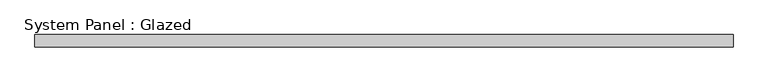
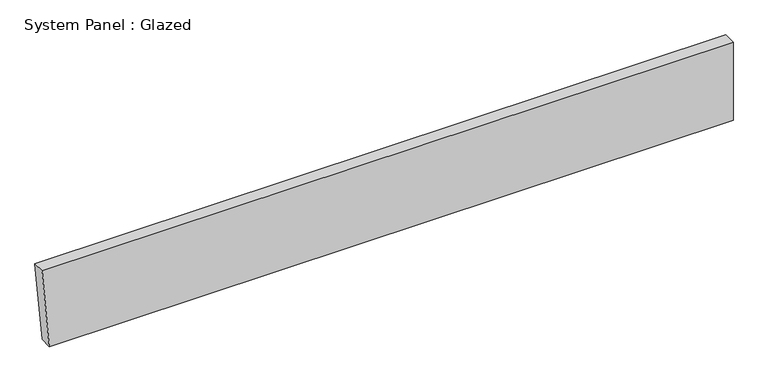
"""IFC4 building model written with IfcOpenShell, lengths in millimetres: plate geometry, System Panel : Glazed."""

from ifc_helpers import new_model, si_unit, frame, origin, place, context, project, spatial, polyline, outline, extrude, source, transform, mapped, element, save


def system_panel_glazed_d86b06c2(model_context):
    return source(origin(), model_context, "Body", "SweptSolid", [
        extrude(outline(polyline([(0.0, -694.0133132), (0.0, 708.5978036), (169.2731269, 708.5978036), (169.2731269, -708.5978036), (0.0, -694.0133132)])), frame((0.0, -44.45, 0.0), z_axis=(0.0, 1.0, 0.0), x_axis=(0.0, 0.0, 1.0)), (0.0, 0.0, 1.0), 25.4),
    ])


if __name__ == "__main__":
    model = new_model("IFC4")
    model_context = context("Model", 3, world=origin())
    ifc_project = project(units=[si_unit("LENGTHUNIT", "METRE", prefix="MILLI")], contexts=[model_context])
    site = spatial("IfcSite", under=ifc_project)
    building = spatial("IfcBuilding", under=site)
    placement = place(None, origin())
    system_panel_glazed_shape = system_panel_glazed_d86b06c2(model_context)
    element("IfcPlate", 1, ObjectType="System Panel : Glazed", at=placement, inside=building, context=model_context, shape_type="MappedRepresentation", body=[
        mapped(system_panel_glazed_shape, transform((0.0, 0.0, 0.0), x_axis=(1.0, 0.0, 0.0), y_axis=(0.0, 1.0, 0.0), z_axis=(0.0, 0.0, 1.0))),
    ])
    save(model, "model.ifc")

# Revit data of these elements
# Type "System Panel : Glazed"
#   Construction Type Id = "GSP4R"
#   Analytic Construction = "1/8 in Pilkington single glazing"
#   Visual Light Transmittance = 0.9
#   Solar Heat Gain Coefficient = 0.86
#   Heat Transfer Coefficient (U) = 1.18115 BTU/(h·ft²·°F)
#   Define Thermal Properties by = 1
# Element 1 (IfcPlate, "System Panel : Glazed")
#   Materials on its faces: "Glass"
# Materials
#   "Glass": class "Glass", colour RGB 0 128 192, transparency 0.75, Description = "Soda Lime Glass", Cost = 0
